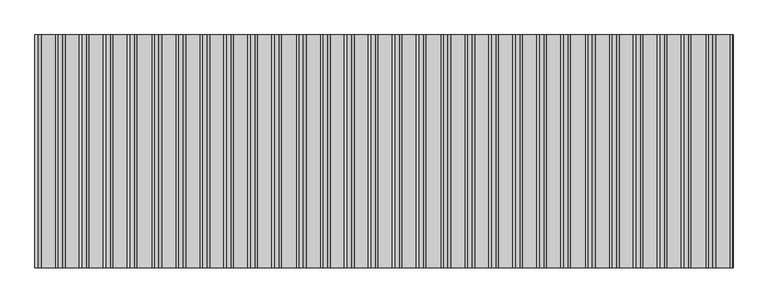
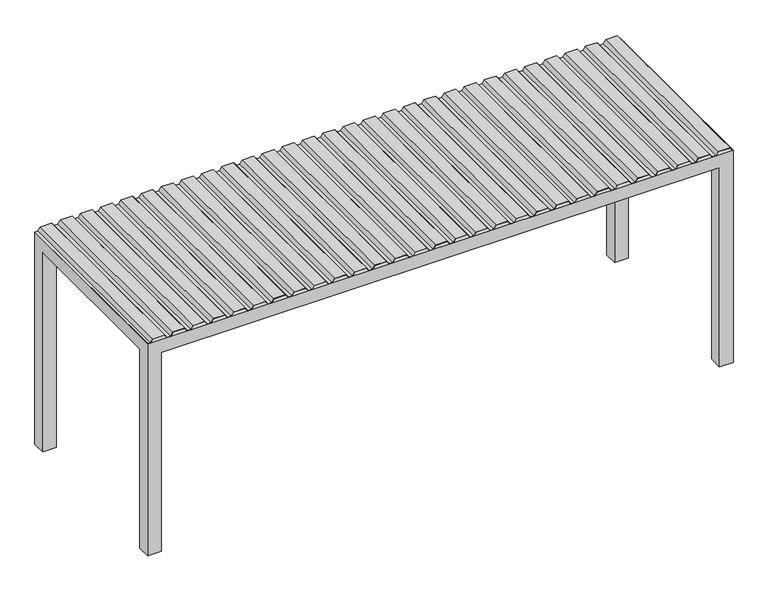
"""IFC4 building model written with IfcOpenShell, lengths in millimetres: proxy geometry, NLRS_90_GM_WPB_fietsenstalling-open_gen_rsf : fietsenstalling bxd 6000x2000mm."""

from ifc_helpers import new_model, si_unit, frame, origin, place, context, project, spatial, polyline, outline, extrude, faceted_brep, source, transform, mapped, element, save


def generic_models_a46722be(model_context):
    return source(origin(), model_context, "Body", "SolidModel", [
        extrude(outline(polyline([(2335.0, -2946.0022315), (2335.0, -2826.9992824), (2300.0, -2803.0007176), (2300.0, -2763.0007963), (2335.0, -2739.0022315), (2335.0, -2619.9992824), (2300.0, -2596.0007176), (2300.0, -2556.0007963), (2335.0, -2532.0022315), (2335.0, -2412.9992824), (2300.0, -2389.0007176), (2300.0, -2349.0007963), (2335.0, -2325.0022315), (2335.0, -2205.9992824), (2300.0, -2182.0007176), (2300.0, -2142.0007963), (2335.0, -2118.0022315), (2335.0, -1998.9992824), (2300.0, -1975.0007176), (2300.0, -1934.9987283), (2335.0, -1911.0001636), (2335.0, -1791.9972144), (2300.0, -1767.9986497), (2300.0, -1727.9987283), (2335.0, -1704.0001636), (2335.0, -1584.9972144), (2300.0, -1560.9986497), (2300.0, -1520.9987283), (2335.0, -1497.0001636), (2335.0, -1377.9972144), (2300.0, -1353.9986497), (2300.0, -1313.9987283), (2335.0, -1290.0001636), (2335.0, -1170.9972144), (2300.0, -1146.9986497), (2300.0, -1106.9987283), (2335.0, -1083.0001636), (2335.0, -963.9972144), (2300.0, -939.9986497), (2300.0, -899.9966604), (2335.0, -875.9980957), (2335.0, -756.9951465), (2300.0, -732.9965818), (2300.0, -692.9966604), (2335.0, -668.9980957), (2335.0, -549.9951465), (2300.0, -525.9965818), (2300.0, -485.9966604), (2335.0, -461.9980957), (2335.0, -342.9951465), (2300.0, -318.9965818), (2300.0, -278.9966604), (2335.0, -254.9980957), (2335.0, -135.9951465), (2300.0, -111.9965818), (2300.0, -71.9966604), (2335.0, -47.9980957), (2335.0, 71.0048535), (2300.0, 95.0034182), (2300.0, 135.0054075), (2335.0, 159.0039722), (2335.0, 278.0069214), (2300.0, 302.0054861), (2300.0, 342.0054075), (2335.0, 366.0039722), (2335.0, 485.0069214), (2300.0, 509.0054861), (2300.0, 549.0054075), (2335.0, 573.0039722), (2335.0, 692.0069214), (2300.0, 716.0054861), (2300.0, 756.0054075), (2335.0, 780.0039722), (2335.0, 899.0069214), (2300.0, 923.0054861), (2300.0, 963.0054075), (2335.0, 987.0039722), (2335.0, 1106.0069214), (2300.0, 1130.0054861), (2300.0, 1170.0074754), (2335.0, 1194.0060401), (2335.0, 1313.0089893), (2300.0, 1337.007554), (2300.0, 1377.0074754), (2335.0, 1401.0060401), (2335.0, 1520.0089893), (2300.0, 1544.007554), (2300.0, 1584.0074754), (2335.0, 1608.0060401), (2335.0, 1727.0089893), (2300.0, 1751.007554), (2300.0, 1791.0074754), (2335.0, 1815.0060401), (2335.0, 1934.0089893), (2300.0, 1958.007554), (2300.0, 1998.0074754), (2335.0, 2022.0060401), (2335.0, 2141.0089893), (2300.0, 2165.007554), (2300.0, 2205.0095433), (2335.0, 2229.008108), (2335.0, 2348.0110572), (2300.0, 2372.0096219), (2300.0, 2412.0095433), (2335.0, 2436.008108), (2335.0, 2555.0110572), (2300.0, 2579.0096219), (2300.0, 2619.0095433), (2335.0, 2643.008108), (2335.0, 2762.0110572), (2300.0, 2786.0096219), (2300.0, 2826.0095433), (2335.0, 2850.008108), (2335.0, 2969.0110572), (2300.0, 2993.0096219), (2300.0, 3000.0), (2302.0, 3000.0), (2302.0, 2994.0632684), (2337.0, 2970.0647037), (2337.0, 2848.9544615), (2302.0, 2824.9558968), (2302.0, 2787.0632684), (2337.0, 2763.0647037), (2337.0, 2641.9544615), (2302.0, 2617.9558968), (2302.0, 2580.0632684), (2337.0, 2556.0647037), (2337.0, 2434.9544615), (2302.0, 2410.9558968), (2302.0, 2373.0632684), (2337.0, 2349.0647037), (2337.0, 2227.9544615), (2302.0, 2203.9558968), (2302.0, 2166.0612005), (2337.0, 2142.0626358), (2337.0, 2020.9523936), (2302.0, 1996.9538289), (2302.0, 1959.0612005), (2337.0, 1935.0626358), (2337.0, 1813.9523936), (2302.0, 1789.9538289), (2302.0, 1752.0612005), (2337.0, 1728.0626358), (2337.0, 1606.9523936), (2302.0, 1582.9538289), (2302.0, 1545.0612005), (2337.0, 1521.0626358), (2337.0, 1399.9523936), (2302.0, 1375.9538289), (2302.0, 1338.0612005), (2337.0, 1314.0626358), (2337.0, 1192.9523936), (2302.0, 1168.9538289), (2302.0, 1131.0591326), (2337.0, 1107.0605679), (2337.0, 985.9503257), (2302.0, 961.951761), (2302.0, 924.0591326), (2337.0, 900.0605679), (2337.0, 778.9503257), (2302.0, 754.951761), (2302.0, 717.0591326), (2337.0, 693.0605679), (2337.0, 571.9503257), (2302.0, 547.951761), (2302.0, 510.0591326), (2337.0, 486.0605679), (2337.0, 364.9503257), (2302.0, 340.951761), (2302.0, 303.0591326), (2337.0, 279.0605679), (2337.0, 157.9503257), (2302.0, 133.951761), (2302.0, 96.0570647), (2337.0, 72.0585), (2337.0, -49.0517422), (2302.0, -73.0503069), (2302.0, -110.9429353), (2337.0, -134.9415), (2337.0, -256.0517422), (2302.0, -280.0503069), (2302.0, -317.9429353), (2337.0, -341.9415), (2337.0, -463.0517422), (2302.0, -487.0503069), (2302.0, -524.9429353), (2337.0, -548.9415), (2337.0, -670.0517422), (2302.0, -694.0503069), (2302.0, -731.9429353), (2337.0, -755.9415), (2337.0, -877.0517422), (2302.0, -901.0503069), (2302.0, -938.9450032), (2337.0, -962.9435679), (2337.0, -1084.0538101), (2302.0, -1108.0523749), (2302.0, -1145.9450032), (2337.0, -1169.9435679), (2337.0, -1291.0538101), (2302.0, -1315.0523749), (2302.0, -1352.9450032), (2337.0, -1376.9435679), (2337.0, -1498.0538101), (2302.0, -1522.0523749), (2302.0, -1559.9450032), (2337.0, -1583.9435679), (2337.0, -1705.0538101), (2302.0, -1729.0523749), (2302.0, -1766.9450032), (2337.0, -1790.9435679), (2337.0, -1912.0538101), (2302.0, -1936.0523749), (2302.0, -1973.9470711), (2337.0, -1997.9456358), (2337.0, -2119.055878), (2302.0, -2143.0544428), (2302.0, -2180.9470711), (2337.0, -2204.9456358), (2337.0, -2326.055878), (2302.0, -2350.0544428), (2302.0, -2387.9470711), (2337.0, -2411.9456358), (2337.0, -2533.055878), (2302.0, -2557.0544428), (2302.0, -2594.9470711), (2337.0, -2618.9456358), (2337.0, -2740.055878), (2302.0, -2764.0544428), (2302.0, -2801.9470711), (2337.0, -2825.9456358), (2337.0, -2947.055878), (2302.0, -2971.0544428), (2302.0, -3000.0), (2300.0, -3000.0), (2300.0, -2970.0007963), (2335.0, -2946.0022315)])), frame((0.0, -1000.0, 0.0), z_axis=(0.0, 1.0, 0.0), x_axis=(0.0, 0.0, 1.0)), (0.0, 0.0, 1.0), 2000.0),
        faceted_brep([(-2860.0, -1000.0, 0.0), (-3000.0, -1000.0, 0.0), (-3000.0, -860.0, 0.0), (-2860.0, -860.0, 0.0), (-2860.0, 860.0, 0.0), (-3000.0, 860.0, 0.0), (-3000.0, 1000.0, 0.0), (-2860.0, 1000.0, 0.0), (3000.0, -1000.0, 0.0), (2860.0, -1000.0, 0.0), (2860.0, -860.0, 0.0), (3000.0, -860.0, 0.0), (3000.0, 860.0, 0.0), (2860.0, 860.0, 0.0), (2860.0, 1000.0, 0.0), (3000.0, 1000.0, 0.0), (-2860.0, -1000.0, 2160.0), (2860.0, -1000.0, 2160.0), (3000.0, -1000.0, 2300.0), (-3000.0, -1000.0, 2300.0), (-3000.0, 1000.0, 2300.0), (-3000.0, 860.0, 2160.0), (-3000.0, -860.0, 2160.0), (-2860.0, -860.0, 2160.0), (-2860.0, 860.0, 2160.0), (3000.0, 1000.0, 2300.0), (2860.0, 1000.0, 2160.0), (-2860.0, 1000.0, 2160.0), (2860.0, -860.0, 2160.0), (3000.0, -860.0, 2160.0), (3000.0, 860.0, 2160.0), (2860.0, 860.0, 2160.0), (2860.0, -860.0, 2300.0), (-2860.0, -860.0, 2300.0), (-2860.0, 860.0, 2300.0), (2860.0, 860.0, 2300.0), (2860.0, 860.0, 2223.0), (2860.0, -860.0, 2223.0), (-2860.0, 860.0, 2223.0), (-2860.0, -860.0, 2223.0)], [[[0, 1, 2, 3]], [[4, 5, 6, 7]], [[8, 9, 10, 11]], [[12, 13, 14, 15]], [[0, 16, 17, 9, 8, 18, 19, 1]], [[19, 20, 6, 5, 21, 22, 2, 1]], [[2, 22, 23, 3]], [[3, 23, 16, 0]], [[4, 24, 21, 5]], [[20, 25, 15, 14, 26, 27, 7, 6]], [[7, 27, 24, 4]], [[9, 17, 28, 10]], [[10, 28, 29, 11]], [[11, 29, 30, 12, 15, 25, 18, 8]], [[12, 30, 31, 13]], [[13, 31, 26, 14]], [[18, 25, 20, 19], [32, 33, 34, 35]], [[23, 22, 21, 24]], [[24, 27, 26, 31]], [[28, 17, 16, 23]], [[31, 30, 29, 28]], [[35, 36, 31, 28, 37, 32]], [[34, 38, 24, 31, 36, 35]], [[33, 39, 23, 24, 38, 34]], [[32, 37, 28, 23, 39, 33]]]),
    ])


if __name__ == "__main__":
    model = new_model("IFC4")
    model_context = context("Model", 3, world=origin())
    ifc_project = project(units=[si_unit("LENGTHUNIT", "METRE", prefix="MILLI")], contexts=[model_context])
    site = spatial("IfcSite", under=ifc_project)
    building = spatial("IfcBuilding", under=site)
    placement = place(None, origin())
    generic_models_shape = generic_models_a46722be(model_context)
    element("IfcBuildingElementProxy", 1, Name="NLRS_90_GM_WPB_fietsenstalling-open_gen_rsf : fietsenstalling bxd 6000x2000mm", ObjectType="NLRS_90_GM_WPB_fietsenstalling-open_gen_rsf : fietsenstalling bxd 6000x2000mm", at=placement, inside=building, context=model_context, shape_type="MappedRepresentation", body=[
        mapped(generic_models_shape, transform((0.0, 0.0, 0.0), x_axis=(1.0, 0.0, 0.0), y_axis=(0.0, 1.0, 0.0), z_axis=(0.0, 0.0, 1.0))),
    ])
    save(model, "model.ifc")

# Revit data of these elements
# Type "NLRS_90_GM_WPB_fietsenstalling-open_gen_rsf : fietsenstalling bxd 6000x2000mm"
#   Type IFC Predefined Type = "USERDEFINED"
#   Export Type to IFC As = "IfcGeographicElementType"
#   Type IfcGUID = "1jnPA0m7n0IPwpoVFqywHL"
#   IfcName[Type] = "fietsenstalling bxd 6000x2000mm"
#   IfcDescription[Type] = "fietsenstalling open bxdxh 6000x2000x2300mm"
#   IfcObjectType[Type] = "BICYCLE_STORAGE"
#   NLRS_C_omschrijving_01 [instance default] = "dak"
#   NLRS_C_omschrijving [instance default] = "constructie"
#   NLRS_C_materiaal_afwerking_01 [instance default] = ""
#   NLRS_C_materiaal_afwerking [instance default] = ""
#   Model = "generiek"
#   Manufacturer = "generiek"
#   Description = "fietsenstalling open bxdxh 6000x2000x2300mm"
#   Assembly Code = "90.22"
#   constructie_dikte = 140.00 mm
#   NLRS_S_gewicht [instance default] = 0.00 kg
#   NLRS_C_oppervlakte = 12.00 m²
#   NLRS_C_hoogte = 2300.00 mm
#   NLRS_C_diepte = 2000.00 mm
#   NLRS_C_breedte = 6000.00 mm
#   Default Elevation = 1219.20 mm
#   NLRS_C_buiten [instance default] = yes
#   NLRS_C_materiaal_01 = none
#   NLRS_C_materiaal = none
#   URL = ""
